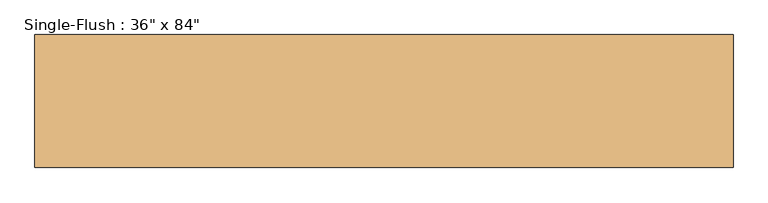
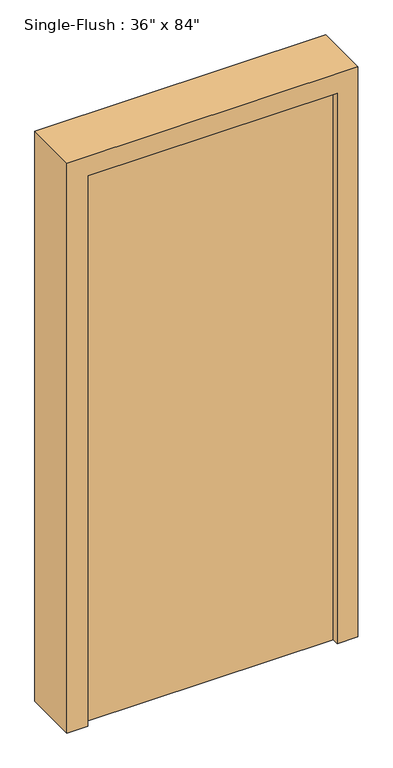
"""IFC4 building model written with IfcOpenShell, lengths in millimetres: door geometry."""

from ifc_helpers import new_model, si_unit, frame, origin, origin_with_axes, place, context, project, spatial, polyline, outline, extrude, source, transform, mapped, element, save


def door_983db92c(model_context):
    return source(origin(), model_context, "Body", "SweptSolid", [
        extrude(outline(polyline([(2209.8, 533.4), (2209.8, -533.4), (0.0, -533.4), (0.0, -457.2), (2133.6, -457.2), (2133.6, 457.2), (0.0, 457.2), (0.0, 533.4), (2209.8, 533.4)])), frame((0.0, -101.6, 0.0), z_axis=(0.0, 1.0, 0.0), x_axis=(0.0, 0.0, 1.0)), (0.0, 0.0, 1.0), 203.2),
        extrude(outline(polyline([(457.2, -25.4), (457.2, -76.2), (-457.2, -76.2), (-457.2, -25.4), (457.2, -25.4)])), origin_with_axes(), (0.0, 0.0, 1.0), 2133.6),
    ])


if __name__ == "__main__":
    model = new_model("IFC4")
    model_context = context("Model", 3, world=origin())
    ifc_project = project(units=[si_unit("LENGTHUNIT", "METRE", prefix="MILLI")], contexts=[model_context])
    site = spatial("IfcSite", under=ifc_project)
    building = spatial("IfcBuilding", under=site)
    placement = place(None, origin())
    door_shape = door_983db92c(model_context)
    element("IfcDoor", 1, ObjectType="Single-Flush : 36\" x 84\"", at=placement, inside=building, context=model_context, shape_type="MappedRepresentation", body=[
        mapped(door_shape, transform((0.0, 0.0, 0.0), x_axis=(1.0, 0.0, 0.0), y_axis=(0.0, 1.0, 0.0), z_axis=(0.0, 0.0, 1.0))),
    ])
    save(model, "model.ifc")

# Revit data of these elements
# Type "Single-Flush : 36\" x 84\""
#   Type Mark = "40"
#   Construction Type Id = "MDOOR"
#   Assembly Code = "C1020"
#   Analytic Construction = "Metal"
#   Thickness = 0' - 2"
#   Thermal Resistance (R) = 0.270117 (m²·K)/W
#   Heat Transfer Coefficient (U) = 3.7021 W/(m²·K)
#   Height = 7' - 0"
#   Trim Projection Ext = 0' - 1"
#   Trim Projection Int = 0' - 1"
#   Trim Width = 0' - 3"
#   Width = 3' - 0"
#   Door Material = Door - Panel
#   Frame Material = Door - Frame
#   Visual Light Transmittance = 0
#   Solar Heat Gain Coefficient = 0
#   Function = (empty or 0)
#   Wall Closure = (empty or 0)
# Element 1 (IfcDoor, "Single-Flush : 36\" x 84\"")
#   Materials on its faces: "Door - Frame", "Door - Panel"
# Materials
#   "Door - Panel": class "Wood", colour RGB 212 179 113, transparency 0, Cost = 0
#   "Door - Frame": class "Miscellaneous", colour RGB 65 65 65, transparency 0, Cost = 0
